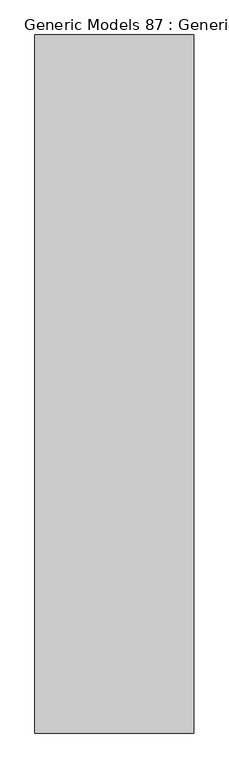
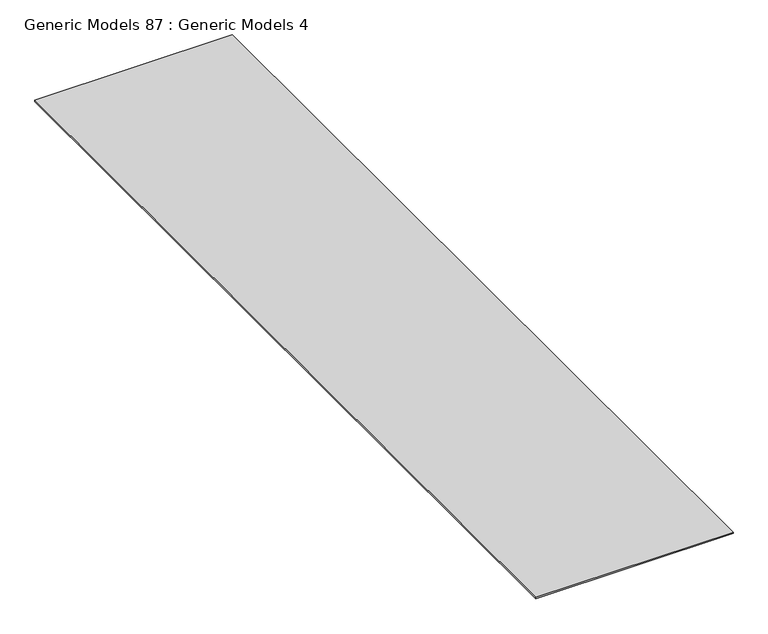
"""IFC4 building model written with IfcOpenShell, lengths in millimetres: proxy geometry, Generic Models 87 : Generic Models 4."""

from ifc_helpers import new_model, si_unit, frame, origin, place, context, project, spatial, polyline, outline, extrude, source, transform, mapped, element, save


def generic_models_87_generic_models_4_68f989a3(model_context):
    return source(origin(), model_context, "Body", "SweptSolid", [
        extrude(outline(polyline([(-6629.5736296, -464.1230338), (-8338.8286276, -464.1230338), (-8338.8286276, 7054.2769662), (-6629.5736296, 7054.2769662), (-6629.5736296, -464.1230338)])), frame((0.0, 0.0, 126361.571), z_axis=(0.0, 0.0, 1.0), x_axis=(1.0, 0.0, 0.0)), (0.0, 0.0, 1.0), 12.7),
    ])


if __name__ == "__main__":
    model = new_model("IFC4")
    model_context = context("Model", 3, world=origin())
    ifc_project = project(units=[si_unit("LENGTHUNIT", "METRE", prefix="MILLI")], contexts=[model_context])
    site = spatial("IfcSite", under=ifc_project)
    building = spatial("IfcBuilding", under=site)
    placement = place(None, origin())
    generic_models_87_generic_models_4_shape = generic_models_87_generic_models_4_68f989a3(model_context)
    element("IfcBuildingElementProxy", 1, Name="Generic Models 87 : Generic Models 4", ObjectType="Generic Models 87 : Generic Models 4", at=placement, inside=building, context=model_context, shape_type="MappedRepresentation", body=[
        mapped(generic_models_87_generic_models_4_shape, transform((0.0, 0.0, 0.0), x_axis=(1.0, 0.0, 0.0), y_axis=(0.0, 1.0, 0.0), z_axis=(0.0, 0.0, 1.0))),
    ])
    save(model, "model.ifc")

# Revit data of these elements
# Element 1 (IfcBuildingElementProxy, "Generic Models 87 : Generic Models 4")
#   Materials on its faces: "_1/2\" CDX PLYWOOD"
# Materials
#   "_1/2\" CDX PLYWOOD": class "Generic", colour RGB 98 75 74, transparency 0, Cost = 0
